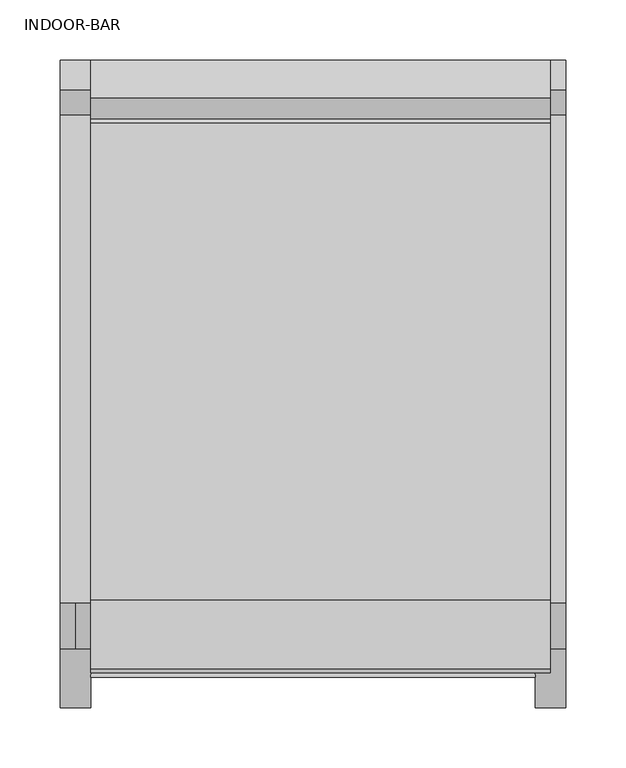
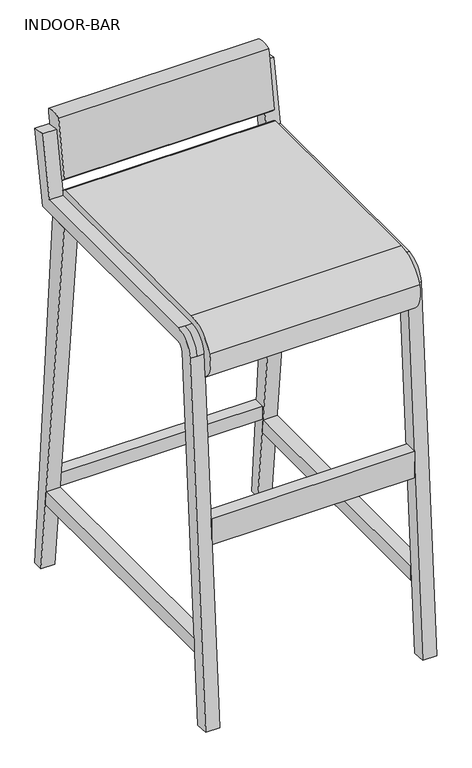
"""IFC4 building model written with IfcOpenShell, lengths in millimetres: furniture geometry, Bar_Stool_6722[1]1 : INDOOR-BAR."""

from ifc_helpers import new_model, si_unit, point, frame, frame_2d, origin, place, context, project, spatial, polyline, circle_curve, trimmed, segment, composite_curve, outline, extrude, source, transform, mapped, element, save
from ifc_brep_helpers import plane_surface, cylinder_surface, revolved_surface, advanced_brep


def indoor_bar_9d95edac(model_context):
    return source(origin(), model_context, "Body", "SolidModel", [
        advanced_brep(
        [(419.1, -25.0141169, 838.4759165), (419.1, 0.0, 834.0652528), (393.7, 0.0, 834.0652528), (393.7, -25.0141169, 838.4759165), (393.7, -45.2169423, 723.9), (419.1, -45.2169423, 723.9), (393.7, -23.9038117, 698.5), (393.7, -450.0350637, 698.5), (393.7, -462.7032819, 686.6979128), (393.7, -511.439502, -0.8979128), (393.7, -536.7759384, 0.8979128), (393.7, -488.0397183, 688.4937383), (393.7, -450.0350637, 723.9), (419.1, -23.9038117, 698.5), (419.1, -450.0350637, 723.9), (419.1, -488.0397183, 688.4937383), (419.1, -536.7759384, 0.8979128), (419.1, -511.439502, -0.8979128), (419.1, -462.7032819, 686.6979128), (419.1, -450.0350637, 698.5), (406.4, -450.0350637, 723.9), (406.4, -488.0397183, 688.4937383)],
        [
            (0, 1),
            (1, 2),
            (2, 3),
            (3, 0),
            (3, 4),
            (4, 5),
            (5, 0),
            (2, 6),
            (6, 7),
            (7, 8, circle_curve(frame((393.7, -450.0350637, 685.8), z_axis=(1.0, 0.0, 0.0), x_axis=(0.0, 0.0, 1.0)), 12.7)),
            (8, 9),
            (9, 10),
            (10, 11),
            (11, 12, circle_curve(frame((393.7, -450.0350637, 685.8), z_axis=(-1.0, 0.0, 0.0), x_axis=(0.0, 0.0, 1.0)), 38.1)),
            (12, 4),
            (1, 13),
            (13, 6),
            (5, 14),
            (14, 15, circle_curve(frame((419.1, -450.0350637, 685.8), z_axis=(1.0, 0.0, 0.0), x_axis=(0.0, 0.0, 1.0)), 38.1)),
            (15, 16),
            (16, 17),
            (17, 18),
            (18, 19, circle_curve(frame((419.1, -450.0350637, 685.8), z_axis=(-1.0, 0.0, 0.0), x_axis=(0.0, 0.0, 1.0)), 12.7)),
            (19, 13),
            (12, 20),
            (20, 14),
            (19, 7),
            (21, 15),
            (20, 21, circle_curve(frame((406.4, -450.0350637, 685.8), z_axis=(1.0, 0.0, 0.0), x_axis=(0.0, 0.0, 1.0)), 38.1)),
            (11, 21),
            (18, 8),
            (10, 16),
            (17, 9),
        ],
        [
            plane_surface(frame((406.4, -12.5070585, 836.2705846), z_axis=(0.0, 0.17364817766692853, 0.9848077530122085), x_axis=(1.0, 0.0, 0.0))),
            plane_surface(frame((406.4, -25.0141169, 838.4759165), z_axis=(0.0, -0.9848077530122085, 0.17364817766692814), x_axis=(0.0, -0.17364817766692814, -0.9848077530122085))),
            plane_surface(frame((393.7, -25.0141169, 838.4759165), z_axis=(-1.0, 0.0, 0.0), x_axis=(0.0, -0.17364817766692808, -0.9848077530122085))),
            plane_surface(frame((393.7, 0.0, 834.0652528), z_axis=(0.0, 0.9848077530122085, -0.17364817766692817), x_axis=(0.0, -0.17364817766692817, -0.9848077530122085))),
            plane_surface(frame((419.1, 0.0, 834.0652528), z_axis=(1.0000000000000002, 0.0, 0.0), x_axis=(0.0, -0.1736481776669284, -0.9848077530122085))),
            plane_surface(frame((406.4, -45.2169423, 723.9), z_axis=(0.0, 0.0, 1.0), x_axis=(0.0, -1.0, 0.0))),
            plane_surface(frame((393.7, -23.9038117, 698.5), z_axis=(0.0, 0.0, -1.0), x_axis=(0.0, -1.0, 0.0))),
            cylinder_surface(frame((406.4, -450.0350637, 685.8), z_axis=(-1.0, 0.0, 0.0), x_axis=(0.0, 0.0, 1.0)), 38.1),
            revolved_surface(polyline([(393.7, -450.0350637, 698.5), (419.1, -450.0350637, 698.5)]), (406.4, -450.0350637, 685.8), (-1.0, 0.0, 0.0)),
            plane_surface(frame((406.4, -488.0397183, 688.4937383), z_axis=(0.0, -0.9974974969901172, 0.07070179275273744), x_axis=(0.0, -0.07070179275273744, -0.9974974969901172))),
            plane_surface(frame((393.7, -462.7032819, 686.6979128), z_axis=(0.0, 0.9974974969901172, -0.07070179275273743), x_axis=(0.0, -0.07070179275273743, -0.9974974969901172))),
            plane_surface(frame((406.4, -524.1077202, 0.0), z_axis=(0.0, -0.07070179275273399, -0.9974974969901175), x_axis=(1.0, 0.0, 0.0))),
        ],
        [
            (0, [[1, 2, 3, 4]]),
            (1, [[-4, 5, 6, 7]]),
            (2, [[8, 9, 10, 11, 12, 13, 14, 15, -5, -3]]),
            (3, [[16, 17, -8, -2]]),
            (4, [[-7, 18, 19, 20, 21, 22, 23, 24, -16, -1]]),
            (5, [[-15, 25, 26, -18, -6]]),
            (6, [[-24, 27, -9, -17]]),
            (7, [[28, -19, -26, 29]]),
            (7, [[30, -29, -25, -14]]),
            (8, [[31, -10, -27, -23]]),
            (9, [[32, -20, -28, -30, -13]]),
            (10, [[33, -11, -31, -22]]),
            (11, [[-12, -33, -21, -32]]),
        ],
    ),
        extrude(outline(composite_curve([segment(polyline([(-48.4096386, 756.5644068), (-31.5225381, 863.1853632)]), True, "CONTINUOUS"), segment(trimmed(circle_curve(frame_2d((-15.7612691, 828.3540875)), 38.2313401), [point((-31.5225381, 863.1853632))], [point((0.0, 863.1853632))], False, "CARTESIAN"), True, "CONTINUOUS"), segment(polyline([(0.0, 863.1853632), (0.0, 856.8353632), (-19.1416957, 748.2774126), (-44.0710693, 752.2258375), (-48.4096386, 756.5644068)]), True, "CONTINUOUS")], self_intersect=False)), frame((25.4, 0.0, 0.0), z_axis=(1.0, 0.0, 0.0), x_axis=(0.0, 1.0, 0.0)), (0.0, 0.0, 1.0), 381.0),
        extrude(outline(composite_curve([segment(polyline([(-51.6744261, 737.5144068), (-43.9498561, 733.0546243), (-46.417441, 704.85), (-452.817441, 704.85), (-460.5585493, 681.23302), (-460.5585493, 643.13302), (-484.2663236, 640.1699505)]), True, "CONTINUOUS"), segment(trimmed(circle_curve(frame_2d((-460.5585493, 681.23302)), 47.4155486), [point((-484.2663236, 640.1699505))], [point((-505.1145904, 697.4500928))], False, "CARTESIAN"), True, "CONTINUOUS"), segment(trimmed(circle_curve(frame_2d((-447.8968201, 676.6245275)), 60.8898793), [point((-505.1145904, 697.4500928))], [point((-447.8968201, 737.5144068))], False, "CARTESIAN"), True, "CONTINUOUS"), segment(polyline([(-447.8968201, 737.5144068), (-51.6744261, 737.5144068)]), True, "CONTINUOUS")], self_intersect=False)), frame((25.4, 0.0, 0.0), z_axis=(1.0, 0.0, 0.0), x_axis=(0.0, 1.0, 0.0)), (0.0, 0.0, 1.0), 381.0),
        extrude(outline(polyline([(393.7, -11.6871233), (393.7, -33.1441574), (25.4, -33.1441574), (25.4, -11.6871233), (393.7, -11.6871233)])), frame((0.0, 0.0, 157.9619127), z_axis=(0.0, 0.0, 1.0), x_axis=(1.0, 0.0, 0.0)), (0.0, 0.0, 1.0), 25.4),
        extrude(outline(polyline([(393.7, -488.2695397), (393.7, -511.439502), (25.4, -511.439502), (25.4, -488.2695397), (393.7, -488.2695397)])), frame((0.0, 0.0, 335.7619127), z_axis=(0.0, 0.0, 1.0), x_axis=(1.0, 0.0, 0.0)), (0.0, 0.0, 1.0), 50.8),
        extrude(outline(polyline([(-500.1796497, 157.9619127), (-35.652466, 157.9619127), (-32.9828185, 132.5619127), (-500.1796497, 132.5619127), (-500.1796497, 157.9619127)])), frame((393.7, 0.0, 0.0), z_axis=(1.0, 0.0, 0.0), x_axis=(0.0, 1.0, 0.0)), (0.0, 0.0, 1.0), 25.4),
        extrude(outline(polyline([(-500.1796497, 157.9619127), (-35.652466, 157.9619127), (-32.9828185, 132.5619127), (-500.1796497, 132.5619127), (-500.1796497, 157.9619127)])), frame((0.0, 0.0, 0.0), z_axis=(1.0, 0.0, 0.0), x_axis=(0.0, 1.0, 0.0)), (0.0, 0.0, 1.0), 25.4),
        extrude(outline(polyline([(0.0, 0.0), (-19.05, 0.0), (-92.4653083, 698.5), (-55.3031462, 698.5), (0.0, 0.0)])), frame((393.7, 0.0, 0.0), z_axis=(1.0, 0.0, 0.0), x_axis=(0.0, 1.0, 0.0)), (0.0, 0.0, 1.0), 25.4),
        advanced_brep(
        [(25.4, -25.0141169, 838.4759165), (25.4, 0.0, 834.0652528), (0.0, 0.0, 834.0652528), (0.0, -25.0141169, 838.4759165), (0.0, -45.2169423, 723.9), (25.4, -45.2169423, 723.9), (0.0, -23.9038117, 698.5), (0.0, -450.0350637, 698.5), (0.0, -462.7032819, 686.6979128), (0.0, -511.439502, -0.8979128), (0.0, -536.7759384, 0.8979128), (0.0, -488.0397183, 688.4937383), (0.0, -450.0350637, 723.9), (25.4, -23.9038117, 698.5), (25.4, -450.0350637, 723.9), (25.4, -488.0397183, 688.4937383), (25.4, -536.7759384, 0.8979128), (25.4, -511.439502, -0.8979128), (25.4, -462.7032819, 686.6979128), (25.4, -450.0350637, 698.5), (12.7, -450.0350637, 723.9), (12.7, -488.0397183, 688.4937383)],
        [
            (0, 1),
            (1, 2),
            (2, 3),
            (3, 0),
            (3, 4),
            (4, 5),
            (5, 0),
            (2, 6),
            (6, 7),
            (7, 8, circle_curve(frame((0.0, -450.0350637, 685.8), z_axis=(1.0, 0.0, 0.0), x_axis=(0.0, 0.0, 1.0)), 12.7)),
            (8, 9),
            (9, 10),
            (10, 11),
            (11, 12, circle_curve(frame((0.0, -450.0350637, 685.8), z_axis=(-1.0, 0.0, 0.0), x_axis=(0.0, 0.0, 1.0)), 38.1)),
            (12, 4),
            (1, 13),
            (13, 6),
            (5, 14),
            (14, 15, circle_curve(frame((25.4, -450.0350637, 685.8), z_axis=(1.0, 0.0, 0.0), x_axis=(0.0, 0.0, 1.0)), 38.1)),
            (15, 16),
            (16, 17),
            (17, 18),
            (18, 19, circle_curve(frame((25.4, -450.0350637, 685.8), z_axis=(-1.0, 0.0, 0.0), x_axis=(0.0, 0.0, 1.0)), 12.7)),
            (19, 13),
            (12, 20),
            (20, 14),
            (19, 7),
            (21, 15),
            (20, 21, circle_curve(frame((12.7, -450.0350637, 685.8), z_axis=(1.0, 0.0, 0.0), x_axis=(0.0, 0.0, 1.0)), 38.1)),
            (11, 21),
            (18, 8),
            (10, 16),
            (17, 9),
        ],
        [
            plane_surface(frame((12.7, -12.5070585, 836.2705846), z_axis=(0.0, 0.17364817766692853, 0.9848077530122085), x_axis=(1.0, 0.0, 0.0))),
            plane_surface(frame((12.7, -25.0141169, 838.4759165), z_axis=(0.0, -0.9848077530122085, 0.173648177666928), x_axis=(0.0, -0.173648177666928, -0.9848077530122085))),
            plane_surface(frame((0.0, -25.0141169, 838.4759165), z_axis=(-1.0, 0.0, 0.0), x_axis=(0.0, -0.17364817766692875, -0.9848077530122084))),
            plane_surface(frame((0.0, 0.0, 834.0652528), z_axis=(0.0, 0.9848077530122084, -0.17364817766692883), x_axis=(0.0, -0.17364817766692883, -0.9848077530122084))),
            plane_surface(frame((25.4, 0.0, 834.0652528), z_axis=(1.0000000000000002, 0.0, 0.0), x_axis=(0.0, -0.1736481776669284, -0.9848077530122085))),
            plane_surface(frame((12.7, -45.2169423, 723.9), z_axis=(0.0, 0.0, 1.0), x_axis=(0.0, -1.0, 0.0))),
            plane_surface(frame((0.0, -23.9038117, 698.5), z_axis=(0.0, 0.0, -1.0), x_axis=(0.0, -1.0, 0.0))),
            cylinder_surface(frame((12.7, -450.0350637, 685.8), z_axis=(-1.0, 0.0, 0.0), x_axis=(0.0, 0.0, 1.0)), 38.1),
            revolved_surface(polyline([(0.0, -450.0350637, 698.5), (25.4, -450.0350637, 698.5)]), (12.7, -450.0350637, 685.8), (-1.0, 0.0, 0.0)),
            plane_surface(frame((12.7, -488.0397183, 688.4937383), z_axis=(0.0, -0.9974974969901172, 0.07070179275273744), x_axis=(0.0, -0.07070179275273744, -0.9974974969901172))),
            plane_surface(frame((0.0, -462.7032819, 686.6979128), z_axis=(0.0, 0.9974974969901172, -0.07070179275273743), x_axis=(0.0, -0.07070179275273743, -0.9974974969901172))),
            plane_surface(frame((12.7, -524.1077202, 0.0), z_axis=(0.0, -0.07070179275273399, -0.9974974969901175), x_axis=(1.0, 0.0, 0.0))),
        ],
        [
            (0, [[1, 2, 3, 4]]),
            (1, [[-4, 5, 6, 7]]),
            (2, [[8, 9, 10, 11, 12, 13, 14, 15, -5, -3]]),
            (3, [[16, 17, -8, -2]]),
            (4, [[-7, 18, 19, 20, 21, 22, 23, 24, -16, -1]]),
            (5, [[-15, 25, 26, -18, -6]]),
            (6, [[-24, 27, -9, -17]]),
            (7, [[28, -19, -26, 29]]),
            (7, [[30, -29, -25, -14]]),
            (8, [[31, -10, -27, -23]]),
            (9, [[32, -20, -28, -30, -13]]),
            (10, [[33, -11, -31, -22]]),
            (11, [[-12, -33, -21, -32]]),
        ],
    ),
        extrude(outline(polyline([(0.0, 0.0), (-19.05, 0.0), (-92.4653083, 698.5), (-55.3031462, 698.5), (0.0, 0.0)])), frame((0.0, 0.0, 0.0), z_axis=(1.0, 0.0, 0.0), x_axis=(0.0, 1.0, 0.0)), (0.0, 0.0, 1.0), 25.4),
    ])


if __name__ == "__main__":
    model = new_model("IFC4")
    model_context = context("Model", 3, world=origin())
    ifc_project = project(units=[si_unit("LENGTHUNIT", "METRE", prefix="MILLI")], contexts=[model_context])
    site = spatial("IfcSite", under=ifc_project)
    building = spatial("IfcBuilding", under=site)
    placement = place(None, origin())
    indoor_bar_shape = indoor_bar_9d95edac(model_context)
    element("IfcFurniture", 1, ObjectType="Bar_Stool_6722[1]1 : INDOOR-BAR", at=placement, inside=building, context=model_context, shape_type="MappedRepresentation", body=[
        mapped(indoor_bar_shape, transform((0.0, 0.0, 0.0), x_axis=(1.0, 0.0, 0.0), y_axis=(0.0, 1.0, 0.0), z_axis=(0.0, 0.0, 1.0))),
    ])
    save(model, "model.ifc")

# Revit data of these elements
# Type "Bar_Stool_6722[1]1 : INDOOR-BAR"
#   Type Mark = "TYPE-BAR"
#   Seating Count = 1
#   Seat = fab
#   Chair Legs = MET
# Element 1 (IfcFurniture, "Bar_Stool_6722[1]1 : INDOOR-BAR")
#   Materials on its faces: "MET", "fab"
# Materials
#   "fab": class "Leather", colour RGB 255 255 255, transparency 0, Cost = 0
#   "MET": class "Metal", colour RGB 189 187 185, transparency 0
